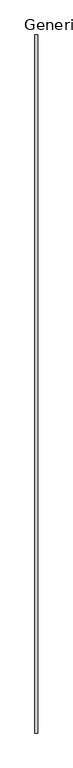
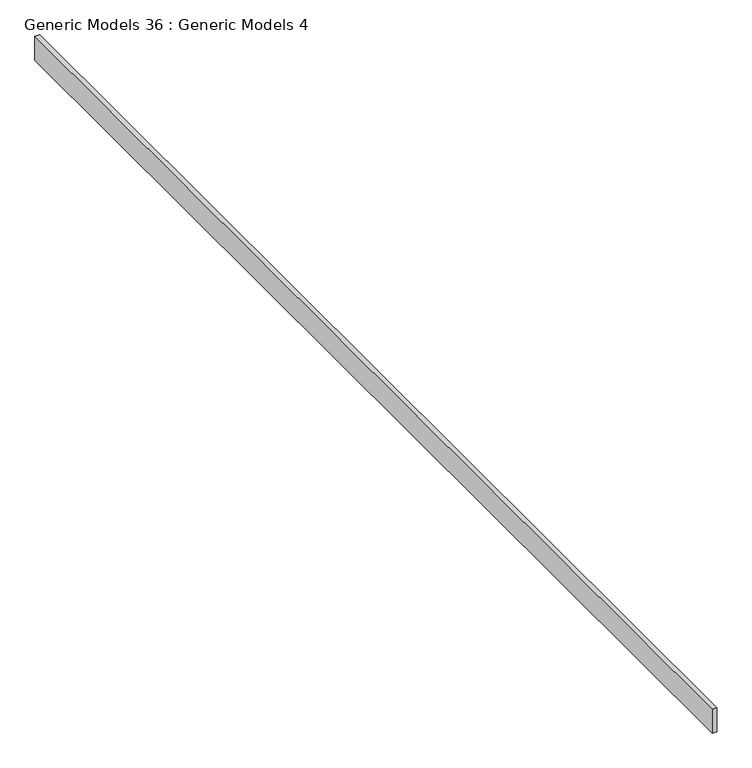
"""IFC4 building model written with IfcOpenShell, lengths in millimetres: proxy geometry, Generic Models 36 : Generic Models 4."""

from ifc_helpers import new_model, si_unit, frame, origin, place, context, project, spatial, polyline, outline, extrude, source, transform, mapped, element, save


def generic_models_36_generic_models_4_7b447f65(model_context):
    return source(origin(), model_context, "Body", "SweptSolid", [
        extrude(outline(polyline([(-9296.3189707, 7054.2769662), (-9315.3689707, 7054.2769662), (-9315.3689707, 11778.6769662), (-9296.3189707, 11778.6769662), (-9296.3189707, 7054.2769662)])), frame((0.0, 0.0, 125494.1987804), z_axis=(0.0, 0.0, 1.0), x_axis=(1.0, 0.0, 0.0)), (0.0, 0.0, 1.0), 101.6),
    ])


if __name__ == "__main__":
    model = new_model("IFC4")
    model_context = context("Model", 3, world=origin())
    ifc_project = project(units=[si_unit("LENGTHUNIT", "METRE", prefix="MILLI")], contexts=[model_context])
    site = spatial("IfcSite", under=ifc_project)
    building = spatial("IfcBuilding", under=site)
    placement = place(None, origin())
    generic_models_36_generic_models_4_shape = generic_models_36_generic_models_4_7b447f65(model_context)
    element("IfcBuildingElementProxy", 1, Name="Generic Models 36 : Generic Models 4", ObjectType="Generic Models 36 : Generic Models 4", at=placement, inside=building, context=model_context, shape_type="MappedRepresentation", body=[
        mapped(generic_models_36_generic_models_4_shape, transform((0.0, 0.0, 0.0), x_axis=(1.0, 0.0, 0.0), y_axis=(0.0, 1.0, 0.0), z_axis=(0.0, 0.0, 1.0))),
    ])
    save(model, "model.ifc")

# Revit data of these elements
# Element 1 (IfcBuildingElementProxy, "Generic Models 36 : Generic Models 4")
#   Materials on its faces: "_CDX PLYWOOD - SEE STRUCT DWGs"
# Materials
#   "_CDX PLYWOOD - SEE STRUCT DWGs": class "Generic", colour RGB 98 75 74, transparency 0, Cost = 0
